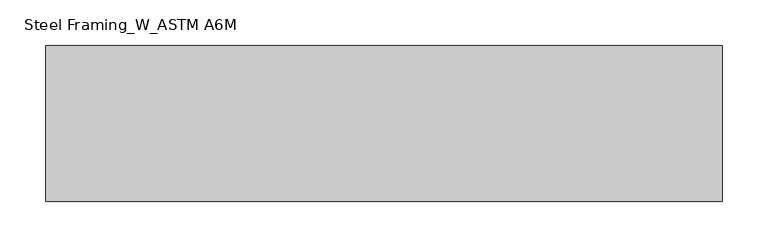
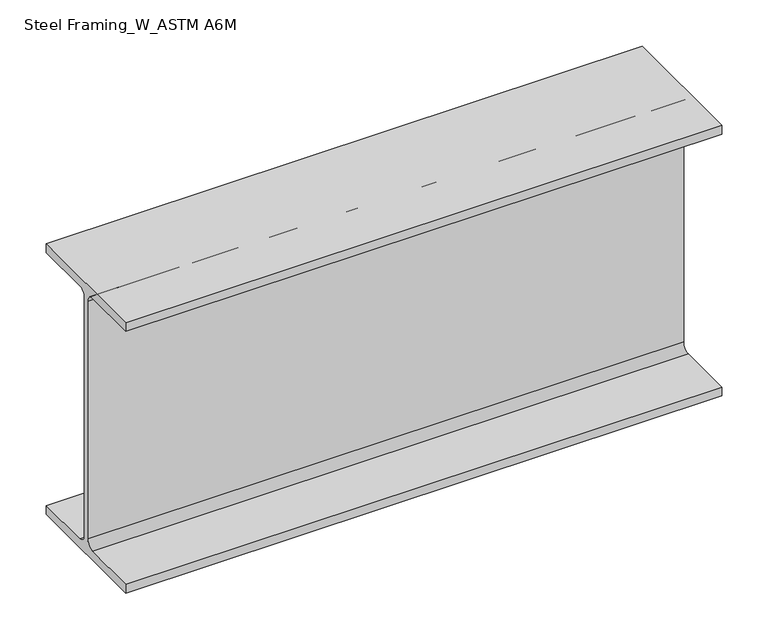
"""IFC4 building model written with IfcOpenShell, lengths in millimetres: beam geometry, Steel Framing_W_ASTM A6M : H_SB_AR_S02_W360x51_RG1."""

from ifc_helpers import new_model, si_unit, point, frame, frame_2d, origin, place, context, project, spatial, polyline, circle_curve, trimmed, segment, composite_curve, outline, extrude, source, transform, mapped, element, save


def steel_framing_w_astm_a6m_9ad73fbe(model_context):
    return source(origin(), model_context, "Body", "SweptSolid", [
        extrude(outline(composite_curve([segment(polyline([(85.5, -166.4), (85.5, -178.0), (-85.5, -178.0), (-85.5, -166.4), (-13.72, -166.4)]), True, "CONTINUOUS"), segment(trimmed(circle_curve(frame_2d((-13.72, -156.3)), 10.1), [point((-13.72, -166.4))], [point((-3.62, -156.3))], True, "CARTESIAN"), True, "CONTINUOUS"), segment(polyline([(-3.62, -156.3), (-3.62, 156.3)]), True, "CONTINUOUS"), segment(trimmed(circle_curve(frame_2d((-13.72, 156.3)), 10.1), [point((-3.62, 156.3))], [point((-13.72, 166.4))], True, "CARTESIAN"), True, "CONTINUOUS"), segment(polyline([(-13.72, 166.4), (-85.5, 166.4), (-85.5, 178.0), (85.5, 178.0), (85.5, 166.4), (13.72, 166.4)]), True, "CONTINUOUS"), segment(trimmed(circle_curve(frame_2d((13.72, 156.3)), 10.1), [point((13.72, 166.4))], [point((3.62, 156.3))], True, "CARTESIAN"), True, "CONTINUOUS"), segment(polyline([(3.62, 156.3), (3.62, -156.3)]), True, "CONTINUOUS"), segment(trimmed(circle_curve(frame_2d((13.72, -156.3)), 10.1), [point((3.62, -156.3))], [point((13.72, -166.4))], True, "CARTESIAN"), True, "CONTINUOUS"), segment(polyline([(13.72, -166.4), (85.5, -166.4)]), True, "CONTINUOUS")], self_intersect=False)), frame((-492.05, 0.0, 0.0), z_axis=(1.0, 0.0, 0.0), x_axis=(0.0, 1.0, 0.0)), (0.0, 0.0, 1.0), 741.4),
    ])


if __name__ == "__main__":
    model = new_model("IFC4")
    model_context = context("Model", 3, world=origin())
    ifc_project = project(units=[si_unit("LENGTHUNIT", "METRE", prefix="MILLI")], contexts=[model_context])
    site = spatial("IfcSite", under=ifc_project)
    building = spatial("IfcBuilding", under=site)
    placement = place(None, origin())
    steel_framing_w_astm_a6m_shape = steel_framing_w_astm_a6m_9ad73fbe(model_context)
    element("IfcBeam", 1, ObjectType="Steel Framing_W_ASTM A6M : H_SB_AR_S02_W360x51_RG1", at=placement, inside=building, context=model_context, shape_type="MappedRepresentation", body=[
        mapped(steel_framing_w_astm_a6m_shape, transform((0.0, 0.0, 0.0), x_axis=(1.0, 0.0, 0.0), y_axis=(0.0, 1.0, 0.0), z_axis=(0.0, 0.0, 1.0))),
    ])
    save(model, "model.ifc")

# Revit data of these elements
# Type "Steel Framing_W_ASTM A6M : H_SB_AR_S02_W360x51_RG1"
#   Type Mark = "RG1"
#   Section Name Key = "W14x34"
#   Width = 17.1 cm
#   Web Thickness = 0.724 cm
#   Web Fillet = 1.01 cm
#   Warping Constant = 287000.0 cm⁶
#   Torsional Moment of Inertia = 23.70 cm⁴
#   Section Area = 64.5 cm²
#   Plastic Modulus weak axis = 174.0 cm³
#   Plastic Modulus strong axis = 895.0 cm³
#   Perimeter = 1.36 m²/m
#   Nominal Weight = 51.00 kgf/m
#   Moment of Inertia weak axis = 970.00 cm⁴
#   Moment of Inertia strong axis = 14200.00 cm⁴
#   Height = 35.6 cm
#   Flange Thickness = 1.16 cm
#   Elastic Modulus weak axis = 113.0 cm³
#   Elastic Modulus strong axis = 796.0 cm³
#   Centroid Vertical = 17.8 cm
#   Centroid Horizontal = 8.55 cm
#   Length [instance default] = 1500 mm
#   Structural Material [instance default] = Steel, 45-345
#   Bolt Spacing = 0
#   Assembly Code = ""
# Element 1 (IfcBeam, "Steel Framing_W_ASTM A6M : H_SB_AR_S02_W360x51_RG1")
#   Materials on its faces: "Steel, 45-345"
# Materials
#   "Steel, 45-345": class "Metal", colour RGB 189 187 185, transparency 0, Description = "Steel 345 MPa", Cost = 0
